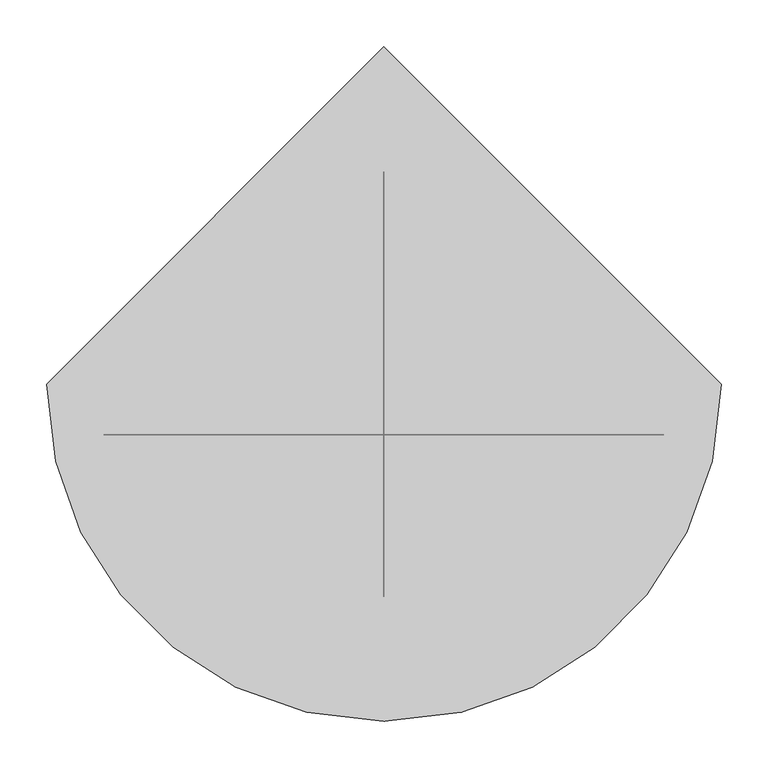
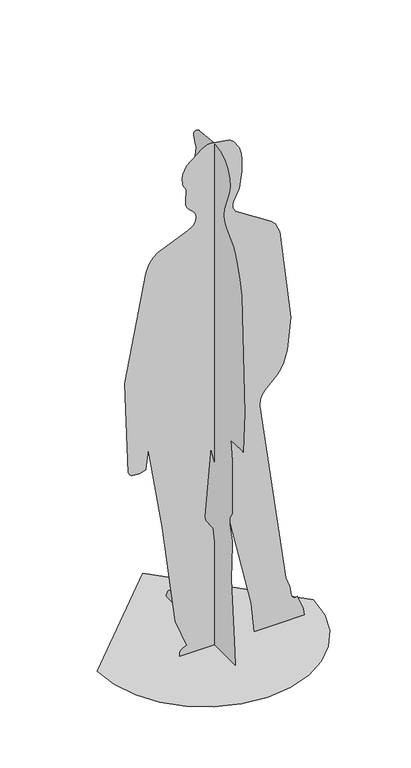
"""IFC4 building model written with IfcOpenShell, lengths in millimetres: proxy geometry, alex 23800 : alex 23800."""

from ifc_helpers import new_model, si_unit, origin, place, context, project, spatial, triangles, source, transform, mapped, element, save


def entourage_2e3e706b(model_context):
    return source(origin(), model_context, "Body", "Tessellation", [
        triangles([(-117.149826, -54.2192196, 0.0), (-117.1651776, -54.2192196, 5.9668874), (-116.2257182, -54.2192196, 11.2908329), (-114.1990069, -54.2192196, 16.0246146), (-110.9487965, -54.2192196, 20.2200526), (-106.3426369, -54.2192196, 23.9299256), (-92.5232224, -54.2192196, 30.1060089), (-131.4701638, -54.2192196, 129.0202679), (-175.160493, -54.2192196, 475.7580242), (-222.3821928, -54.2192196, 767.9406984), (-230.1656384, -54.2192196, 699.5134071), (-235.7141188, -54.2192196, 696.8034708), (-252.8135111, -54.2192196, 693.0705591), (-271.5672719, -54.2192196, 693.4227905), (-279.1847031, -54.2192196, 695.8179932), (-284.3598959, -54.2192196, 700.0603941), (-288.7942909, -54.2192196, 709.0155161), (-300.0380995, -54.2192196, 1027.779562), (-230.6060912, -54.2192196, 1391.1560738), (-226.4231343, -54.2192196, 1402.4037884), (-221.6912647, -54.2192196, 1413.4720081), (-216.4584809, -54.2192196, 1423.8837273), (-210.7698928, -54.2192196, 1433.1671722), (-204.6734626, -54.2192196, 1440.846936), (-189.6343552, -54.2192196, 1451.6253479), (-89.8842756, -54.2192196, 1494.9825851), (-71.747551, -54.2192196, 1507.2129433), (-63.0092944, -54.2192196, 1520.5333511), (-61.6725528, -54.2192196, 1534.6925159), (-63.8671908, -54.2192196, 1545.3268959), (-68.585621, -54.2192196, 1553.4059086), (-87.7951952, -54.2192196, 1572.0070988), (-92.5232224, -54.2192196, 1579.5592541), (-95.9145034, -54.2192196, 1589.6919205), (-97.2061397, -54.2192196, 1598.308255), (-95.4740416, -54.2192196, 1641.5380291), (-96.331938, -54.2192196, 1644.515609), (-97.9843898, -54.2192196, 1647.8886589), (-100.1204967, -54.2192196, 1651.4987583), (-102.4302848, -54.2192196, 1655.1874866), (-104.5999834, -54.2192196, 1658.7975861), (-106.3205724, -54.2192196, 1662.170636), (-107.2792258, -54.2192196, 1665.1483612), (-108.4230876, -54.2192196, 1683.4309662), (-105.9731918, -54.2192196, 1699.5698067), (-100.5907078, -54.2192196, 1713.7231579), (-92.9406569, -54.2192196, 1726.0522018), (-41.9073575, -54.2192196, 1768.6831753), (-23.8378028, -54.2192196, 1776.4340103), (-13.1083444, -54.2192196, 1778.0000484), (45.7765254, -54.2192196, 1768.297443), (52.0927142, -54.2192196, 1765.4942711), (63.2559182, -54.2192196, 1755.9912174), (81.7812909, -54.2192196, 1728.0616722), (88.745219, -54.2192196, 1704.6000229), (91.0789973, -54.2192196, 1685.137112), (90.9475373, -54.2192196, 1642.2940876), (81.6066376, -54.2192196, 1585.4628181), (62.4047392, -54.2192196, 1543.9670952), (60.537325, -54.2192196, 1533.9496834), (60.9470838, -54.2192196, 1523.4841885), (69.4089674, -54.2192196, 1508.7943874), (187.9492836, -54.2192196, 1431.6201736), (202.6112339, -54.2192196, 1417.2355865), (217.8863916, -54.2192196, 1383.1912983), (254.1089989, -54.2192196, 1069.0535688), (242.364258, -54.2192196, 957.3563169), (229.1733843, -54.2192196, 912.5566532), (220.0532106, -54.2192196, 895.7643642), (208.0071618, -54.2192196, 880.6840347), (194.42189, -54.2192196, 866.7791422), (180.6849923, -54.2192196, 853.5153442), (168.1831209, -54.2192196, 840.3571358), (158.3057987, -54.2192196, 826.7670496), (152.4387149, -54.2192196, 812.2106707), (150.4446415, -54.2192196, 791.5933245), (238.0268047, -54.2192196, 154.0623804), (251.6370204, -54.2192196, 116.8321946), (256.996468, -54.2192196, 85.1121104), (259.9472872, -54.2192196, 78.4667766), (263.4038167, -54.2192196, 74.733874), (267.3257794, -54.2192196, 73.2493489), (271.6699546, -54.2192196, 73.3510687), (276.3951023, -54.2192196, 74.375938), (297.1717229, -54.2192196, 23.3148105), (300.0371367, -54.2192196, 0.0), (131.8280998, -54.2192196, 0.0), (122.3288704, -54.2192196, 103.0617143), (-12.8367732, -54.2192196, 700.0603941), (-32.6518678, -54.2192196, 465.9114232), (-30.5455124, -54.2192196, 452.1476558), (-28.5399163, -54.2192196, 446.8956871), (-9.3111464, -54.2192196, 418.9977533), (-6.9341794, -54.2192196, 413.7803392), (0.9020383, -54.2192196, 348.2760163), (3.9440186, -54.2192196, 338.8305536), (7.6318198, -54.2192196, 329.4100167), (11.5067468, -54.2192196, 320.0537564), (15.1043435, -54.2192196, 310.8021046), (17.965916, -54.2192196, 301.6953567), (20.1922245, -54.2192196, 275.8289304), (9.4637256, -54.2192196, 194.8220472), (10.7735997, -54.2192196, 177.672767), (25.5305637, -54.2192196, 136.3536502), (26.3020941, -54.2192196, 0.0), (0.0, -171.2567705, 45.1949975), (0.0, -150.8745481, 290.639618), (0.0, -156.0132787, 413.7064339), (0.0, -155.0152837, 426.2860439), (0.0, -142.9452446, 479.8709636), (0.0, -142.1842718, 491.5446696), (0.0, -143.2100995, 503.0207133), (0.0, -144.047839, 505.2451052), (0.0, -145.7118181, 508.1738508), (0.0, -147.8757485, 511.5296053), (0.0, -150.2143322, 515.036041), (0.0, -152.400327, 518.4148682), (0.0, -154.109416, 521.3887055), (0.0, -155.0152837, 523.6802808), (0.0, -156.6389491, 713.2963594), (0.0, -149.1126916, 780.4474205), (0.0, -210.0425026, 781.4050655), (0.0, -219.9447689, 780.4474205), (0.0, -227.6802342, 923.8398308), (0.0, -210.5088804, 1326.6335587), (0.0, -200.0250727, 1381.4668396), (0.0, -183.9208231, 1432.731443), (0.0, -173.3612024, 1455.0204895), (0.0, -160.9178849, 1474.0122082), (0.0, -124.7336655, 1511.6876701), (0.0, -116.986691, 1522.764465), (0.0, -111.1138482, 1535.6011814), (0.0, -107.7935748, 1550.7469139), (0.0, -109.4844237, 1573.6183376), (0.0, -138.1807553, 1647.6468132), (0.0, -144.3654704, 1674.2838501), (0.0, -143.232173, 1701.9783806), (0.0, -131.4049152, 1730.7792389), (0.0, -113.8084512, 1751.5885792), (0.0, -93.3149074, 1763.9963974), (0.0, -70.4587898, 1769.8088333), (0.0, -45.7765254, 1770.8327534), (0.0, 33.8705797, 1763.2439724), (0.0, 35.8723357, 1763.9599171), (0.0, 40.3067194, 1762.4466373), (0.0, 46.2419403, 1759.1397171), (0.0, 52.7442914, 1754.4731415), (0.0, 58.882952, 1748.8852558), (0.0, 63.7242081, 1742.8090279), (0.0, 66.3353223, 1736.6819309), (0.0, 66.7661872, 1728.2947975), (0.0, 65.1444384, 1720.0201572), (0.0, 62.192661, 1712.2874897), (0.0, 55.1980298, 1700.1665726), (0.0, 51.5783606, 1695.362796), (0.0, 72.2379144, 1580.2608101), (0.0, 61.7953832, 1563.4866886), (0.0, 54.5483692, 1508.478709), (0.0, -4.4967569, 1482.8666096), (0.0, 4.8441379, 1466.163414), (0.0, 131.2648075, 892.5976244), (0.0, 131.4039524, 884.7393105), (0.0, 130.533584, 877.3195599), (0.0, 128.9799633, 870.382556), (0.0, 127.06649, 863.9703747), (0.0, 125.1175083, 858.1292341), (0.0, 123.4573807, 852.9002655), (0.0, 122.4104424, 848.3277248), (0.0, 121.9344722, 836.2039009), (0.0, 123.662737, 824.5599169), (0.0, 138.1893939, 779.9867655), (0.0, 140.1191817, 768.6412371), (0.0, 134.7798818, 638.2851677), (0.0, 137.1673996, 618.1236803), (0.0, 142.9922621, 588.3899938), (0.0, 150.2623125, 530.9436092), (0.0, 150.5262045, 510.8147143), (0.0, 148.9725838, 491.2155109), (0.0, 104.741045, 115.2804997), (0.0, 107.6544391, 83.9308235), (0.0, 113.0014147, 72.9595455), (0.0, 123.907435, 63.6781489), (0.0, 138.4753594, 55.956123), (0.0, 154.8099183, 49.6658456), (0.0, 171.0159059, 44.676806), (0.0, 185.196145, 40.8613776), (0.0, 195.4573101, 38.0900079), (0.0, 202.9931691, 35.5086429), (0.0, 208.9821204, 32.4772168), (0.0, 213.7648408, 28.6934543), (0.0, 217.6848777, 23.8550755), (0.0, 221.0819088, 17.6607589), (0.0, 224.3004623, 9.8101468), (0.0, 227.6802342, 0.0), (0.0, -172.9495269, 0.0), (-361.2442655, 0.0, 0.0), (-351.6941943, -82.7735268, 0.0), (-324.4958181, -158.787528, 0.0), (-281.8265113, -225.8636845, 0.0), (-225.8646292, -281.8265113, 0.0), (-158.787528, -324.4948371, 0.0), (-82.7735268, -351.6941943, 0.0), (0.0, -361.2442655, 0.0), (82.7735268, -351.6941943, 0.0), (158.787528, -324.4958181, 0.0), (225.8646292, -281.8265113, 0.0), (281.8265113, -225.8636845, 0.0), (324.4958181, -158.787528, 0.0), (351.6941943, -82.7735268, 0.0), (361.2442655, 0.0, 0.0), (0.0, 361.2442655, 0.0)], [[85, 86, 87], [105, 1, 2], [105, 2, 3], [105, 3, 4], [105, 4, 5], [105, 5, 6], [105, 6, 7], [85, 87, 88], [104, 105, 7], [104, 7, 8], [103, 104, 8], [102, 103, 8], [102, 8, 9], [101, 102, 9], [100, 101, 9], [99, 100, 9], [98, 99, 9], [97, 98, 9], [96, 97, 9], [95, 96, 9], [94, 95, 9], [93, 94, 9], [92, 93, 9], [91, 92, 9], [90, 91, 9], [90, 9, 10], [89, 90, 10], [83, 84, 85], [10, 11, 12], [10, 12, 13], [10, 13, 14], [10, 14, 15], [10, 15, 16], [10, 16, 17], [10, 17, 18], [89, 10, 18], [89, 18, 19], [89, 19, 20], [89, 20, 21], [89, 21, 22], [89, 22, 23], [89, 23, 24], [89, 24, 25], [89, 25, 26], [89, 26, 27], [89, 27, 28], [82, 83, 85], [82, 85, 88], [81, 82, 88], [80, 81, 88], [79, 80, 88], [78, 79, 88], [77, 78, 88], [76, 77, 88], [76, 88, 89], [76, 89, 28], [75, 76, 28], [74, 75, 28], [73, 74, 28], [72, 73, 28], [71, 72, 28], [70, 71, 28], [69, 70, 28], [68, 69, 28], [67, 68, 28], [66, 67, 28], [65, 66, 28], [64, 65, 28], [63, 64, 28], [62, 63, 28], [61, 62, 28], [61, 28, 29], [60, 61, 29], [59, 60, 29], [59, 29, 30], [59, 30, 31], [58, 59, 31], [57, 58, 31], [57, 31, 32], [57, 32, 33], [57, 33, 34], [57, 34, 35], [57, 35, 36], [56, 57, 36], [56, 36, 37], [55, 56, 37], [54, 55, 37], [53, 54, 37], [52, 53, 37], [51, 52, 37], [50, 51, 37], [49, 50, 37], [48, 49, 37], [47, 48, 37], [47, 37, 38], [46, 47, 38], [45, 46, 38], [44, 45, 38], [43, 44, 38], [43, 38, 39], [43, 39, 40], [43, 40, 41], [43, 41, 42], [193, 194, 195], [192, 193, 195], [191, 192, 195], [190, 191, 195], [189, 190, 195], [188, 189, 195], [187, 188, 195], [186, 187, 195], [185, 186, 195], [184, 185, 195], [183, 184, 195], [182, 183, 195], [181, 182, 195], [181, 195, 106], [180, 181, 106], [179, 180, 106], [122, 123, 124], [179, 106, 107], [178, 179, 107], [178, 107, 108], [178, 108, 109], [178, 109, 110], [178, 110, 111], [177, 178, 111], [177, 111, 112], [176, 177, 112], [175, 176, 112], [175, 112, 113], [174, 175, 113], [174, 113, 114], [174, 114, 115], [174, 115, 116], [173, 174, 116], [173, 116, 117], [173, 117, 118], [173, 118, 119], [173, 119, 120], [173, 120, 121], [172, 173, 121], [171, 172, 121], [170, 171, 121], [169, 170, 121], [168, 169, 121], [167, 168, 121], [157, 158, 159], [166, 167, 121], [165, 166, 121], [164, 165, 121], [163, 164, 121], [162, 163, 121], [161, 162, 121], [121, 122, 124], [160, 161, 121], [160, 121, 124], [160, 124, 125], [160, 125, 126], [160, 126, 127], [160, 127, 128], [160, 128, 129], [159, 160, 129], [159, 129, 130], [159, 130, 131], [159, 131, 132], [157, 159, 132], [157, 132, 133], [157, 133, 134], [156, 157, 134], [155, 156, 134], [155, 134, 135], [155, 135, 136], [155, 136, 137], [155, 137, 138], [155, 138, 139], [155, 139, 140], [155, 140, 141], [155, 141, 142], [155, 142, 143], [154, 155, 143], [153, 154, 143], [152, 153, 143], [151, 152, 143], [150, 151, 143], [149, 150, 143], [148, 149, 143], [147, 148, 143], [146, 147, 143], [145, 146, 143], [144, 145, 143], [210, 211, 196], [209, 210, 196], [209, 196, 197], [208, 209, 197], [208, 197, 198], [208, 198, 199], [207, 208, 199], [206, 207, 199], [206, 199, 200], [206, 200, 201], [206, 201, 202], [206, 202, 203], [206, 203, 204], [206, 204, 205]], closed=False),
    ])


if __name__ == "__main__":
    model = new_model("IFC4")
    model_context = context("Model", 3, world=origin())
    ifc_project = project(units=[si_unit("LENGTHUNIT", "METRE", prefix="MILLI")], contexts=[model_context])
    site = spatial("IfcSite", under=ifc_project)
    building = spatial("IfcBuilding", under=site)
    placement = place(None, origin())
    entourage_shape = entourage_2e3e706b(model_context)
    element("IfcBuildingElementProxy", 1, Name="alex 23800 : alex 23800", ObjectType="alex 23800 : alex 23800", at=placement, inside=building, context=model_context, shape_type="MappedRepresentation", body=[
        mapped(entourage_shape, transform((0.0, 0.0, 0.0), x_axis=(1.0, 0.0, 0.0), y_axis=(0.0, 1.0, 0.0), z_axis=(0.0, 0.0, 1.0))),
    ])
    save(model, "model.ifc")

# Revit data of these elements
# Type "alex 23800 : alex 23800"
#   built-in parameter 1005195 = "RPC-8-X9C2-NGU9-LXF5-4"
#   Height = 0
